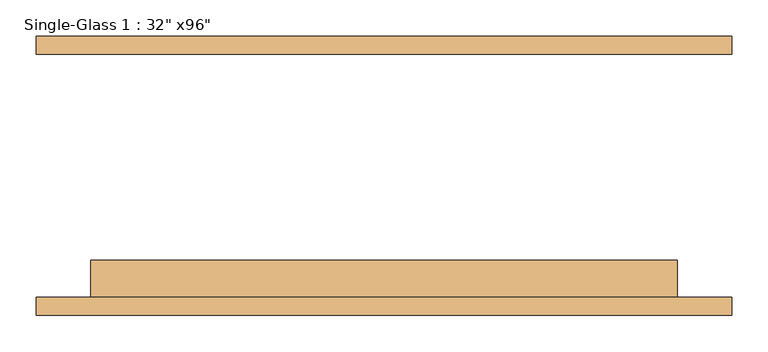
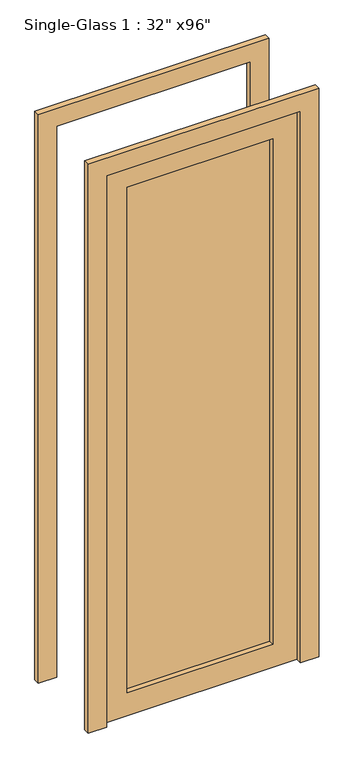
"""IFC4 building model written with IfcOpenShell, lengths in millimetres: door geometry."""

from ifc_helpers import new_model, si_unit, frame, origin, place, context, project, spatial, polyline, outline, extrude, source, transform, mapped, element, save


def door_c6c76292(model_context):
    return source(origin(), model_context, "Body", "SweptSolid", [
        extrude(outline(polyline([(2438.4, 406.4), (0.0, 406.4), (0.0, 482.6), (2514.6, 482.6), (2514.6, -482.6), (0.0, -482.6), (0.0, -406.4), (2438.4, -406.4), (2438.4, 406.4)])), frame((0.0, 168.275, 0.0), z_axis=(0.0, 1.0, 0.0), x_axis=(0.0, 0.0, 1.0)), (0.0, 0.0, 1.0), 25.4),
        extrude(outline(polyline([(2438.4, 406.4), (0.0, 406.4), (0.0, 482.6), (2514.6, 482.6), (2514.6, -482.6), (0.0, -482.6), (0.0, -406.4), (2438.4, -406.4), (2438.4, 406.4)])), frame((0.0, -193.675, 0.0), z_axis=(0.0, 1.0, 0.0), x_axis=(0.0, 0.0, 1.0)), (0.0, 0.0, 1.0), 25.4),
        extrude(outline(polyline([(304.8, -139.7), (304.8, -146.05), (-304.8, -146.05), (-304.8, -139.7), (304.8, -139.7)])), frame((0.0, 0.0, 101.6), z_axis=(0.0, 0.0, 1.0), x_axis=(1.0, 0.0, 0.0)), (0.0, 0.0, 1.0), 2235.2),
        extrude(outline(polyline([(2438.4, 406.4), (2438.4, -406.4), (0.0, -406.4), (0.0, 406.4), (2438.4, 406.4)]), holes=[polyline([(2336.8, -304.8), (2336.8, 304.8), (101.6, 304.8), (101.6, -304.8), (2336.8, -304.8)])]), frame((0.0, -168.275, 0.0), z_axis=(0.0, 1.0, 0.0), x_axis=(0.0, 0.0, 1.0)), (0.0, 0.0, 1.0), 50.8),
    ])


if __name__ == "__main__":
    model = new_model("IFC4")
    model_context = context("Model", 3, world=origin())
    ifc_project = project(units=[si_unit("LENGTHUNIT", "METRE", prefix="MILLI")], contexts=[model_context])
    site = spatial("IfcSite", under=ifc_project)
    building = spatial("IfcBuilding", under=site)
    placement = place(None, origin())
    door_shape = door_c6c76292(model_context)
    element("IfcDoor", 1, ObjectType="Single-Glass 1 : 32\" x96\"", at=placement, inside=building, context=model_context, shape_type="MappedRepresentation", body=[
        mapped(door_shape, transform((0.0, 0.0, 0.0), x_axis=(1.0, 0.0, 0.0), y_axis=(0.0, 1.0, 0.0), z_axis=(0.0, 0.0, 1.0))),
    ])
    save(model, "model.ifc")

# Revit data of these elements
# Type "Single-Glass 1 : 32\" x96\""
#   Type Mark = "31"
#   Construction Type Id = "MDOOR"
#   Assembly Code = "C1020"
#   Analytic Construction = "Metal"
#   Thickness = 0' - 2"
#   Heat Transfer Coefficient (U) = 3.7021 W/(m²·K)
#   Height = 8' - 0"
#   Rail Width - Base = 0' - 4"
#   Rail Width - Top = 0' - 4"
#   Stile Width - Hinge = 0' - 4"
#   Stile Width - Latch = 0' - 4"
#   Trim Projection Ext = 0' - 1"
#   Trim Projection Int = 0' - 1"
#   Trim Width = 0' - 3"
#   Width = 2' - 8"
#   Door Material = Aluminum
#   Frame Material = Aluminum
#   Visual Light Transmittance = 0
#   Solar Heat Gain Coefficient = 0
#   Function = (empty or 0)
#   Wall Closure = (empty or 0)
# Element 1 (IfcDoor, "Single-Glass 1 : 32\" x96\"")
#   Materials on its faces: "Aluminum", "Glass"
# Materials
#   "Aluminum": class "Metal", colour RGB 226 226 226, transparency 0, Description = "Aluminum 6061", Cost = 0
#   "Glass": class "Glass", colour RGB 142 168 196, transparency 0.75, Description = "Soda Lime Glass", Cost = 0
